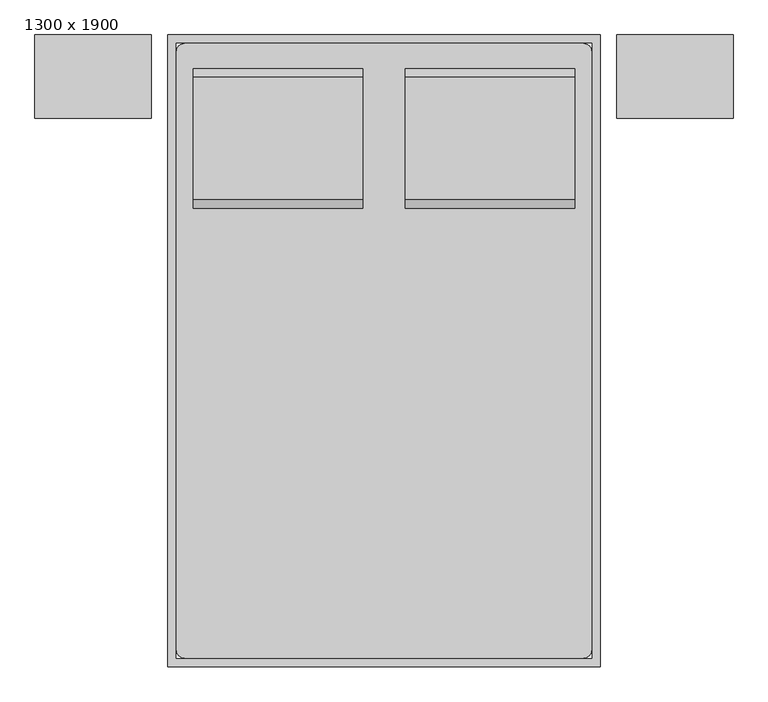
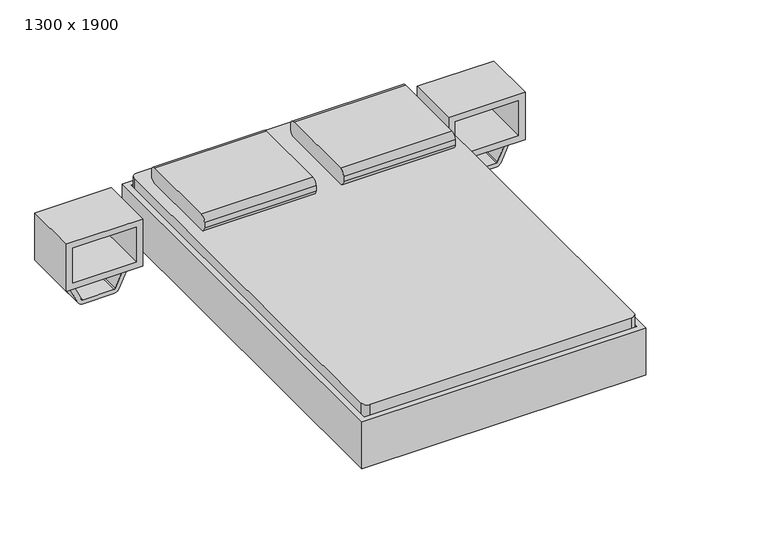
"""IFC4 building model written with IfcOpenShell, lengths in millimetres: furniture geometry, 双人床带床头柜 : 1300 x 1900."""

from ifc_helpers import new_model, si_unit, point, frame, frame_2d, origin, place, context, project, spatial, polyline, circle_curve, trimmed, segment, composite_curve, outline, extrude, source, transform, mapped, element, save
from ifc_brep_helpers import plane_surface, cylinder_surface, revolved_surface, advanced_brep


def furniture_1300_x_1900_48583a1e(model_context):
    return source(origin(), model_context, "Body", "SolidModel", [
        advanced_brep(
        [(-285.1231784, 461.5704918, 177.8), (-285.1231784, 385.3704918, 177.8), (-285.1231784, 385.3704918, 196.85), (-285.1231784, 461.5704918, 196.85), (-234.3231784, 461.5704918, 177.8), (-234.3231784, 385.3704918, 177.8), (-222.1869899, 385.3704918, 196.85), (-222.1869899, 461.5704918, 196.85), (-158.2523099, 461.5704918, 14.6654962), (-158.2523099, 385.3704918, 14.6654962), (-140.9871466, 385.3704918, 22.716374), (-140.9871466, 461.5704918, 22.716374), (-135.2320921, 385.3704918, 0.0), (-135.2320921, 461.5704918, 0.0), (-135.2320921, 385.3704918, 19.05), (-135.2320921, 461.5704918, 19.05), (-56.6195862, 461.5704918, 0.0), (-56.6195862, 385.3704918, 0.0), (-56.6195862, 385.3704918, 19.05), (-56.6195862, 461.5704918, 19.05), (-43.9195862, 385.3704918, 3.4029547), (-43.9195862, 461.5704918, 3.4029547), (-53.4445862, 385.3704918, 19.9007387), (-53.4445862, 461.5704918, 19.9007387), (16.177459, 461.5704918, 38.1), (16.177459, 385.3704918, 38.1), (11.0730269, 385.3704918, 57.15), (11.0730269, 461.5704918, 57.15), (662.4518216, 461.5704918, 38.1), (662.4518216, 385.3704918, 38.1), (667.5562537, 385.3704918, 57.15), (667.5562537, 461.5704918, 57.15), (722.5488669, 461.5704918, 3.4029547), (722.5488669, 385.3704918, 3.4029547), (732.0738669, 385.3704918, 19.9007387), (732.0738669, 461.5704918, 19.9007387), (735.2488669, 385.3704918, 0.0), (735.2488669, 461.5704918, 0.0), (735.2488669, 385.3704918, 19.05), (735.2488669, 461.5704918, 19.05), (813.8613728, 461.5704918, 0.0), (813.8613728, 385.3704918, 0.0), (813.8613728, 385.3704918, 19.05), (813.8613728, 461.5704918, 19.05), (836.8815906, 385.3704918, 14.6654962), (836.8815906, 461.5704918, 14.6654962), (819.6164272, 385.3704918, 22.716374), (819.6164272, 461.5704918, 22.716374), (912.952459, 461.5704918, 177.8), (912.952459, 385.3704918, 177.8), (900.8162705, 385.3704918, 196.85), (900.8162705, 461.5704918, 196.85), (963.752459, 461.5704918, 177.8), (963.752459, 461.5704918, 196.85), (963.752459, 385.3704918, 196.85), (963.752459, 385.3704918, 177.8)],
        [
            (0, 1),
            (1, 2),
            (2, 3),
            (3, 0),
            (0, 4),
            (4, 5),
            (5, 1),
            (5, 6),
            (6, 2),
            (6, 7),
            (7, 3),
            (7, 4),
            (4, 8),
            (8, 9),
            (9, 5),
            (9, 10),
            (10, 6),
            (10, 11),
            (11, 7),
            (11, 8),
            (12, 9, circle_curve(frame((-135.2320921, 385.3704918, 25.4), z_axis=(0.0, 1.0, 0.0), x_axis=(-0.9063077870366494, 0.0, -0.4226182617407007)), 25.4)),
            (8, 13, circle_curve(frame((-135.2320921, 461.5704918, 25.4), z_axis=(0.0, -1.0, 0.0), x_axis=(-0.9063077870366494, 0.0, -0.4226182617407007)), 25.4)),
            (13, 12),
            (14, 10, circle_curve(frame((-135.2320921, 385.3704918, 25.4), z_axis=(0.0, 1.0, 0.0), x_axis=(-0.9063077870366494, 0.0, -0.4226182617407007)), 6.35)),
            (12, 14),
            (15, 11, circle_curve(frame((-135.2320921, 461.5704918, 25.4), z_axis=(0.0, 1.0, 0.0), x_axis=(-0.9063077870366494, 0.0, -0.4226182617407007)), 6.35)),
            (14, 15),
            (15, 13),
            (13, 16),
            (16, 17),
            (17, 12),
            (17, 18),
            (18, 14),
            (18, 19),
            (19, 15),
            (19, 16),
            (20, 17, circle_curve(frame((-56.6195862, 385.3704918, 25.4), z_axis=(0.0, 1.0, 0.0), x_axis=(0.0, 0.0, -1.0)), 25.4)),
            (16, 21, circle_curve(frame((-56.6195862, 461.5704918, 25.4), z_axis=(0.0, -1.0, 0.0), x_axis=(0.0, 0.0, -1.0)), 25.4)),
            (21, 20),
            (22, 18, circle_curve(frame((-56.6195862, 385.3704918, 25.4), z_axis=(0.0, 1.0, 0.0), x_axis=(0.0, 0.0, -1.0)), 6.35)),
            (20, 22),
            (23, 19, circle_curve(frame((-56.6195862, 461.5704918, 25.4), z_axis=(0.0, 1.0, 0.0), x_axis=(0.0, 0.0, -1.0)), 6.35)),
            (22, 23),
            (23, 21),
            (21, 24),
            (24, 25),
            (25, 20),
            (25, 26),
            (26, 22),
            (26, 27),
            (27, 23),
            (27, 24),
            (24, 28),
            (28, 29),
            (29, 25),
            (29, 30),
            (30, 26),
            (30, 31),
            (31, 27),
            (31, 28),
            (28, 32),
            (32, 33),
            (33, 29),
            (33, 34),
            (34, 30),
            (34, 35),
            (35, 31),
            (35, 32),
            (36, 33, circle_curve(frame((735.2488669, 385.3704918, 25.4), z_axis=(0.0, 1.0, 0.0), x_axis=(-0.5000000000000505, 0.0, -0.8660254037844094)), 25.4)),
            (32, 37, circle_curve(frame((735.2488669, 461.5704918, 25.4), z_axis=(0.0, -1.0, 0.0), x_axis=(-0.5000000000000505, 0.0, -0.8660254037844094)), 25.4)),
            (37, 36),
            (38, 34, circle_curve(frame((735.2488669, 385.3704918, 25.4), z_axis=(0.0, 1.0, 0.0), x_axis=(-0.5000000000000505, 0.0, -0.8660254037844094)), 6.35)),
            (36, 38),
            (39, 35, circle_curve(frame((735.2488669, 461.5704918, 25.4), z_axis=(0.0, 1.0, 0.0), x_axis=(-0.5000000000000505, 0.0, -0.8660254037844094)), 6.35)),
            (38, 39),
            (39, 37),
            (37, 40),
            (40, 41),
            (41, 36),
            (41, 42),
            (42, 38),
            (42, 43),
            (43, 39),
            (43, 40),
            (44, 41, circle_curve(frame((813.8613728, 385.3704918, 25.4), z_axis=(0.0, 1.0, 0.0), x_axis=(0.0, 0.0, -1.0)), 25.4)),
            (40, 45, circle_curve(frame((813.8613728, 461.5704918, 25.4), z_axis=(0.0, -1.0, 0.0), x_axis=(0.0, 0.0, -1.0)), 25.4)),
            (45, 44),
            (46, 42, circle_curve(frame((813.8613728, 385.3704918, 25.4), z_axis=(0.0, 1.0, 0.0), x_axis=(0.0, 0.0, -1.0)), 6.35)),
            (44, 46),
            (47, 43, circle_curve(frame((813.8613728, 461.5704918, 25.4), z_axis=(0.0, 1.0, 0.0), x_axis=(0.0, 0.0, -1.0)), 6.35)),
            (46, 47),
            (47, 45),
            (45, 48),
            (48, 49),
            (49, 44),
            (49, 50),
            (50, 46),
            (50, 51),
            (51, 47),
            (51, 48),
            (52, 53),
            (53, 54),
            (54, 55),
            (55, 52),
            (48, 52),
            (55, 49),
            (54, 50),
            (53, 51),
        ],
        [
            plane_surface(frame((-285.1231784, 715.5704918, -152.9490627), z_axis=(-1.0, 0.0, 0.0), x_axis=(0.0, 1.0, 0.0))),
            plane_surface(frame((-285.1231784, 461.5704918, 177.8), z_axis=(0.0, 0.0, -1.0), x_axis=(1.0, 0.0, 0.0))),
            plane_surface(frame((-285.1231784, 385.3704918, 177.8), z_axis=(0.0, -1.0, 0.0), x_axis=(1.0, 0.0, 0.0))),
            plane_surface(frame((-285.1231784, 385.3704918, 196.85), z_axis=(0.0, 0.0, 1.0), x_axis=(1.0, 0.0, 0.0))),
            plane_surface(frame((-285.1231784, 461.5704918, 196.85), z_axis=(0.0, 1.0, 0.0), x_axis=(1.0, 0.0, 0.0))),
            plane_surface(frame((-234.3231784, 461.5704918, 177.8), z_axis=(-0.9063077870366483, 0.0, -0.42261826174070305), x_axis=(0.42261826174070305, 0.0, -0.9063077870366483))),
            plane_surface(frame((-234.3231784, 385.3704918, 177.8), z_axis=(0.0, -1.0, 0.0), x_axis=(0.4226182617407031, 0.0, -0.9063077870366483))),
            plane_surface(frame((-222.1869899, 385.3704918, 196.85), z_axis=(0.9063077870366483, 0.0, 0.42261826174070316), x_axis=(0.42261826174070316, 0.0, -0.9063077870366483))),
            plane_surface(frame((-222.1869899, 461.5704918, 196.85), z_axis=(0.0, 1.0, 0.0), x_axis=(0.42261826174070316, 0.0, -0.9063077870366483))),
            cylinder_surface(frame((-135.2320921, 715.5704918, 25.4), z_axis=(0.0, -1.0, 0.0), x_axis=(-0.9063077870366494, 0.0, -0.4226182617407007)), 25.4),
            plane_surface(frame((-135.2320921, 385.3704918, 25.4), z_axis=(0.0, -1.0, 0.0), x_axis=(-0.9063077870366494, 0.0, -0.4226182617407007))),
            revolved_surface(polyline([(-140.9871465476827, 385.3704918, 22.71637403794655), (-140.9871465476827, 461.5704918, 22.71637403794655)]), (-135.2320921, 715.5704918, 25.4), (0.0, -1.0, 0.0)),
            plane_surface(frame((-135.2320921, 461.5704918, 25.4), z_axis=(0.0, 1.0, 0.0), x_axis=(-0.9063077870366494, 0.0, -0.4226182617407007))),
            plane_surface(frame((-135.2320921, 461.5704918, 0.0), z_axis=(0.0, 0.0, -1.0), x_axis=(1.0, 0.0, 0.0))),
            plane_surface(frame((-135.2320921, 385.3704918, 0.0), z_axis=(0.0, -1.0, 0.0), x_axis=(1.0, 0.0, 0.0))),
            plane_surface(frame((-135.2320921, 385.3704918, 19.05), z_axis=(0.0, 0.0, 1.0), x_axis=(1.0, 0.0, 0.0))),
            plane_surface(frame((-135.2320921, 461.5704918, 19.05), z_axis=(0.0, 1.0, 0.0), x_axis=(1.0, 0.0, 0.0))),
            cylinder_surface(frame((-56.6195862, 715.5704918, 25.4), z_axis=(0.0, -1.0, 0.0), x_axis=(0.0, 0.0, -1.0)), 25.4),
            plane_surface(frame((-56.6195862, 385.3704918, 25.4), z_axis=(0.0, -1.0, 0.0), x_axis=(0.0, 0.0, -1.0))),
            revolved_surface(polyline([(-56.6195862, 385.3704918, 19.049999999999997), (-56.6195862, 461.5704918, 19.049999999999997)]), (-56.6195862, 715.5704918, 25.4), (0.0, -1.0, 0.0)),
            plane_surface(frame((-56.6195862, 461.5704918, 25.4), z_axis=(0.0, 1.0, 0.0), x_axis=(0.0, 0.0, -1.0))),
            plane_surface(frame((-43.9195862, 461.5704918, 3.4029547), z_axis=(0.49999999999987826, 0.0, -0.8660254037845089), x_axis=(0.8660254037845089, 0.0, 0.49999999999987826))),
            plane_surface(frame((-43.9195862, 385.3704918, 3.4029547), z_axis=(0.0, -1.0, 0.0), x_axis=(0.866025403784509, 0.0, 0.49999999999987815))),
            plane_surface(frame((-53.4445862, 385.3704918, 19.9007387), z_axis=(-0.49999999999987926, 0.0, 0.8660254037845083), x_axis=(0.8660254037845083, 0.0, 0.49999999999987926))),
            plane_surface(frame((-53.4445862, 461.5704918, 19.9007387), z_axis=(0.0, 1.0, 0.0), x_axis=(0.8660254037845087, 0.0, 0.4999999999998789))),
            plane_surface(frame((16.177459, 461.5704918, 38.1), z_axis=(0.0, 0.0, -1.0), x_axis=(1.0, 0.0, 0.0))),
            plane_surface(frame((16.177459, 385.3704918, 38.1), z_axis=(0.0, -1.0, 0.0), x_axis=(1.0, 0.0, 0.0))),
            plane_surface(frame((11.0730269, 385.3704918, 57.15), z_axis=(0.0, 0.0, 1.0), x_axis=(1.0, 0.0, 0.0))),
            plane_surface(frame((11.0730269, 461.5704918, 57.15), z_axis=(0.0, 1.0, 0.0), x_axis=(1.0, 0.0, 0.0))),
            plane_surface(frame((662.4518216, 461.5704918, 38.1), z_axis=(-0.5000000000000518, 0.0, -0.8660254037844087), x_axis=(0.8660254037844087, 0.0, -0.5000000000000518))),
            plane_surface(frame((662.4518216, 385.3704918, 38.1), z_axis=(0.0, -1.0, 0.0), x_axis=(0.8660254037844093, 0.0, -0.500000000000051))),
            plane_surface(frame((667.5562537, 385.3704918, 57.15), z_axis=(0.5000000000000507, 0.0, 0.8660254037844094), x_axis=(0.8660254037844094, 0.0, -0.5000000000000507))),
            plane_surface(frame((667.5562537, 461.5704918, 57.15), z_axis=(0.0, 1.0000000000000002, 0.0), x_axis=(0.8660254037844094, 0.0, -0.5000000000000508))),
            cylinder_surface(frame((735.2488669, 715.5704918, 25.4), z_axis=(0.0, -1.0, 0.0), x_axis=(-0.5000000000000505, 0.0, -0.8660254037844094)), 25.4),
            plane_surface(frame((735.2488669, 385.3704918, 25.4), z_axis=(0.0, -1.0, 0.0), x_axis=(-0.5000000000000506, 0.0, -0.8660254037844095))),
            revolved_surface(polyline([(732.0738668999998, 385.3704918, 19.900738685969), (732.0738668999998, 461.5704918, 19.900738685969)]), (735.2488669, 715.5704918, 25.4), (0.0, -1.0, 0.0)),
            plane_surface(frame((735.2488669, 461.5704918, 25.4), z_axis=(0.0, 1.0, 0.0), x_axis=(-0.5000000000000506, 0.0, -0.8660254037844095))),
            plane_surface(frame((735.2488669, 461.5704918, 0.0), z_axis=(0.0, 0.0, -1.0), x_axis=(1.0, 0.0, 0.0))),
            plane_surface(frame((735.2488669, 385.3704918, 0.0), z_axis=(0.0, -1.0, 0.0), x_axis=(1.0, 0.0, 0.0))),
            plane_surface(frame((735.2488669, 385.3704918, 19.05), z_axis=(0.0, 0.0, 1.0), x_axis=(1.0, 0.0, 0.0))),
            plane_surface(frame((735.2488669, 461.5704918, 19.05), z_axis=(0.0, 1.0, 0.0), x_axis=(1.0, 0.0, 0.0))),
            cylinder_surface(frame((813.8613728, 715.5704918, 25.4), z_axis=(0.0, -1.0, 0.0), x_axis=(0.0, 0.0, -1.0)), 25.4),
            plane_surface(frame((813.8613728, 385.3704918, 25.4), z_axis=(0.0, -1.0, 0.0), x_axis=(0.0, 0.0, -1.0))),
            revolved_surface(polyline([(813.8613728, 385.3704918, 19.049999999999997), (813.8613728, 461.5704918, 19.049999999999997)]), (813.8613728, 715.5704918, 25.4), (0.0, -1.0, 0.0)),
            plane_surface(frame((813.8613728, 461.5704918, 25.4), z_axis=(0.0, 1.0, 0.0), x_axis=(0.0, 0.0, -1.0))),
            plane_surface(frame((836.8815906, 461.5704918, 14.6654962), z_axis=(0.9063077870366775, 0.0, -0.42261826174064077), x_axis=(0.42261826174064077, 0.0, 0.9063077870366775))),
            plane_surface(frame((836.8815906, 385.3704918, 14.6654962), z_axis=(0.0, -1.0, 0.0), x_axis=(0.42261826174063993, 0.0, 0.9063077870366777))),
            plane_surface(frame((819.6164272, 385.3704918, 22.716374), z_axis=(-0.9063077870366776, 0.0, 0.4226182617406402), x_axis=(0.4226182617406402, 0.0, 0.9063077870366776))),
            plane_surface(frame((819.6164272, 461.5704918, 22.716374), z_axis=(0.0, 1.0, 0.0), x_axis=(0.4226182617406405, 0.0, 0.9063077870366775))),
            plane_surface(frame((963.752459, 715.5704918, -152.9490627), z_axis=(1.0, 0.0, 0.0), x_axis=(0.0, 1.0, 0.0))),
            plane_surface(frame((912.952459, 461.5704918, 177.8), z_axis=(0.0, 0.0, -1.0), x_axis=(1.0, 0.0, 0.0))),
            plane_surface(frame((912.952459, 385.3704918, 177.8), z_axis=(0.0, -1.0, 0.0), x_axis=(1.0, 0.0, 0.0))),
            plane_surface(frame((900.8162705, 385.3704918, 196.85), z_axis=(0.0, 0.0, 1.0), x_axis=(1.0, 0.0, 0.0))),
            plane_surface(frame((900.8162705, 461.5704918, 196.85), z_axis=(0.0, 1.0, 0.0), x_axis=(1.0, 0.0, 0.0))),
        ],
        [
            (0, [[1, 2, 3, 4]]),
            (1, [[-1, 5, 6, 7]]),
            (2, [[-2, -7, 8, 9]]),
            (3, [[-3, -9, 10, 11]]),
            (4, [[-4, -11, 12, -5]]),
            (5, [[-6, 13, 14, 15]]),
            (6, [[-8, -15, 16, 17]]),
            (7, [[-10, -17, 18, 19]]),
            (8, [[-12, -19, 20, -13]]),
            (9, [[21, -14, 22, 23]]),
            (10, [[24, -16, -21, 25]]),
            (11, [[26, -18, -24, 27]]),
            (12, [[-22, -20, -26, 28]]),
            (13, [[-23, 29, 30, 31]]),
            (14, [[-25, -31, 32, 33]]),
            (15, [[-27, -33, 34, 35]]),
            (16, [[-28, -35, 36, -29]]),
            (17, [[37, -30, 38, 39]]),
            (18, [[40, -32, -37, 41]]),
            (19, [[42, -34, -40, 43]]),
            (20, [[-38, -36, -42, 44]]),
            (21, [[-39, 45, 46, 47]]),
            (22, [[-41, -47, 48, 49]]),
            (23, [[-43, -49, 50, 51]]),
            (24, [[-44, -51, 52, -45]]),
            (25, [[-46, 53, 54, 55]]),
            (26, [[-48, -55, 56, 57]]),
            (27, [[-50, -57, 58, 59]]),
            (28, [[-52, -59, 60, -53]]),
            (29, [[-54, 61, 62, 63]]),
            (30, [[-56, -63, 64, 65]]),
            (31, [[-58, -65, 66, 67]]),
            (32, [[-60, -67, 68, -61]]),
            (33, [[69, -62, 70, 71]]),
            (34, [[72, -64, -69, 73]]),
            (35, [[74, -66, -72, 75]]),
            (36, [[-70, -68, -74, 76]]),
            (37, [[-71, 77, 78, 79]]),
            (38, [[-73, -79, 80, 81]]),
            (39, [[-75, -81, 82, 83]]),
            (40, [[-76, -83, 84, -77]]),
            (41, [[85, -78, 86, 87]]),
            (42, [[88, -80, -85, 89]]),
            (43, [[90, -82, -88, 91]]),
            (44, [[-86, -84, -90, 92]]),
            (45, [[-87, 93, 94, 95]]),
            (46, [[-89, -95, 96, 97]]),
            (47, [[-91, -97, 98, 99]]),
            (48, [[-92, -99, 100, -93]]),
            (49, [[101, 102, 103, 104]]),
            (50, [[-94, 105, -104, 106]]),
            (51, [[-96, -106, -103, 107]]),
            (52, [[-98, -107, -102, 108]]),
            (53, [[-100, -108, -101, -105]]),
        ],
    ),
        advanced_brep(
        [(-285.447541, -879.6295082, 196.85), (-285.447541, -879.6295082, 177.8), (-285.447541, -955.8295082, 177.8), (-285.447541, -955.8295082, 196.85), (-222.5113525, -879.6295082, 196.85), (-234.647541, -879.6295082, 177.8), (-234.647541, -955.8295082, 177.8), (-222.5113525, -955.8295082, 196.85), (-141.3115092, -879.6295082, 22.716374), (-158.5766725, -879.6295082, 14.6654962), (-158.5766725, -955.8295082, 14.6654962), (-141.3115092, -955.8295082, 22.716374), (-135.5564547, -879.6295082, 0.0), (-135.5564547, -879.6295082, 19.05), (-135.5564547, -955.8295082, 0.0), (-135.5564547, -955.8295082, 19.05), (-56.9439489, -879.6295082, 19.05), (-56.9439489, -879.6295082, 0.0), (-56.9439489, -955.8295082, 0.0), (-56.9439489, -955.8295082, 19.05), (-44.2439489, -879.6295082, 3.4029547), (-53.7689489, -879.6295082, 19.9007387), (-44.2439489, -955.8295082, 3.4029547), (-53.7689489, -955.8295082, 19.9007387), (10.7486643, -879.6295082, 57.15), (15.8530964, -879.6295082, 38.1), (15.8530964, -955.8295082, 38.1), (10.7486643, -955.8295082, 57.15), (667.5562537, -879.6295082, 57.15), (662.4518216, -879.6295082, 38.1), (662.4518216, -955.8295082, 38.1), (667.5562537, -955.8295082, 57.15), (732.0738669, -879.6295082, 19.9007387), (722.5488669, -879.6295082, 3.4029547), (722.5488669, -955.8295082, 3.4029547), (732.0738669, -955.8295082, 19.9007387), (735.2488669, -879.6295082, 0.0), (735.2488669, -879.6295082, 19.05), (735.2488669, -955.8295082, 0.0), (735.2488669, -955.8295082, 19.05), (813.8613728, -879.6295082, 19.05), (813.8613728, -879.6295082, 0.0), (813.8613728, -955.8295082, 0.0), (813.8613728, -955.8295082, 19.05), (836.8815906, -879.6295082, 14.6654962), (819.6164272, -879.6295082, 22.716374), (836.8815906, -955.8295082, 14.6654962), (819.6164272, -955.8295082, 22.716374), (900.8162705, -879.6295082, 196.85), (912.952459, -879.6295082, 177.8), (912.952459, -955.8295082, 177.8), (900.8162705, -955.8295082, 196.85), (963.752459, -879.6295082, 196.85), (963.752459, -955.8295082, 196.85), (963.752459, -955.8295082, 177.8), (963.752459, -879.6295082, 177.8)],
        [
            (0, 1),
            (1, 2),
            (2, 3),
            (3, 0),
            (0, 4),
            (4, 5),
            (5, 1),
            (5, 6),
            (6, 2),
            (6, 7),
            (7, 3),
            (7, 4),
            (4, 8),
            (8, 9),
            (9, 5),
            (9, 10),
            (10, 6),
            (10, 11),
            (11, 7),
            (11, 8),
            (12, 9, circle_curve(frame((-135.5564547, -879.6295082, 25.4), z_axis=(0.0, 1.0, 0.0), x_axis=(-0.9063077870366627, 0.0, -0.42261826174067213)), 25.4)),
            (8, 13, circle_curve(frame((-135.5564547, -879.6295082, 25.4), z_axis=(0.0, -1.0, 0.0), x_axis=(-0.9063077870366627, 0.0, -0.42261826174067213)), 6.35)),
            (13, 12),
            (14, 10, circle_curve(frame((-135.5564547, -955.8295082, 25.4), z_axis=(0.0, 1.0, 0.0), x_axis=(-0.9063077870366627, 0.0, -0.42261826174067213)), 25.4)),
            (12, 14),
            (15, 11, circle_curve(frame((-135.5564547, -955.8295082, 25.4), z_axis=(0.0, 1.0, 0.0), x_axis=(-0.9063077870366627, 0.0, -0.42261826174067213)), 6.35)),
            (14, 15),
            (15, 13),
            (13, 16),
            (16, 17),
            (17, 12),
            (17, 18),
            (18, 14),
            (18, 19),
            (19, 15),
            (19, 16),
            (20, 17, circle_curve(frame((-56.9439489, -879.6295082, 25.4), z_axis=(0.0, 1.0, 0.0), x_axis=(0.0, 0.0, -1.0)), 25.4)),
            (16, 21, circle_curve(frame((-56.9439489, -879.6295082, 25.4), z_axis=(0.0, -1.0, 0.0), x_axis=(0.0, 0.0, -1.0)), 6.35)),
            (21, 20),
            (22, 18, circle_curve(frame((-56.9439489, -955.8295082, 25.4), z_axis=(0.0, 1.0, 0.0), x_axis=(0.0, 0.0, -1.0)), 25.4)),
            (20, 22),
            (23, 19, circle_curve(frame((-56.9439489, -955.8295082, 25.4), z_axis=(0.0, 1.0, 0.0), x_axis=(0.0, 0.0, -1.0)), 6.35)),
            (22, 23),
            (23, 21),
            (21, 24),
            (24, 25),
            (25, 20),
            (25, 26),
            (26, 22),
            (26, 27),
            (27, 23),
            (27, 24),
            (24, 28),
            (28, 29),
            (29, 25),
            (29, 30),
            (30, 26),
            (30, 31),
            (31, 27),
            (31, 28),
            (28, 32),
            (32, 33),
            (33, 29),
            (33, 34),
            (34, 30),
            (34, 35),
            (35, 31),
            (35, 32),
            (36, 33, circle_curve(frame((735.2488669, -879.6295082, 25.4), z_axis=(0.0, 1.0, 0.0), x_axis=(-0.5000000000000517, 0.0, -0.8660254037844087)), 25.4)),
            (32, 37, circle_curve(frame((735.2488669, -879.6295082, 25.4), z_axis=(0.0, -1.0, 0.0), x_axis=(-0.5000000000000517, 0.0, -0.8660254037844087)), 6.35)),
            (37, 36),
            (38, 34, circle_curve(frame((735.2488669, -955.8295082, 25.4), z_axis=(0.0, 1.0, 0.0), x_axis=(-0.5000000000000517, 0.0, -0.8660254037844087)), 25.4)),
            (36, 38),
            (39, 35, circle_curve(frame((735.2488669, -955.8295082, 25.4), z_axis=(0.0, 1.0, 0.0), x_axis=(-0.5000000000000517, 0.0, -0.8660254037844087)), 6.35)),
            (38, 39),
            (39, 37),
            (37, 40),
            (40, 41),
            (41, 36),
            (41, 42),
            (42, 38),
            (42, 43),
            (43, 39),
            (43, 40),
            (44, 41, circle_curve(frame((813.8613728, -879.6295082, 25.4), z_axis=(0.0, 1.0, 0.0), x_axis=(0.0, 0.0, -1.0)), 25.4)),
            (40, 45, circle_curve(frame((813.8613728, -879.6295082, 25.4), z_axis=(0.0, -1.0, 0.0), x_axis=(0.0, 0.0, -1.0)), 6.35)),
            (45, 44),
            (46, 42, circle_curve(frame((813.8613728, -955.8295082, 25.4), z_axis=(0.0, 1.0, 0.0), x_axis=(0.0, 0.0, -1.0)), 25.4)),
            (44, 46),
            (47, 43, circle_curve(frame((813.8613728, -955.8295082, 25.4), z_axis=(0.0, 1.0, 0.0), x_axis=(0.0, 0.0, -1.0)), 6.35)),
            (46, 47),
            (47, 45),
            (45, 48),
            (48, 49),
            (49, 44),
            (49, 50),
            (50, 46),
            (50, 51),
            (51, 47),
            (51, 48),
            (52, 53),
            (53, 54),
            (54, 55),
            (55, 52),
            (48, 52),
            (55, 49),
            (54, 50),
            (53, 51),
        ],
        [
            plane_surface(frame((-285.447541, -1184.4295082, -127.5947323), z_axis=(-1.0, 0.0, 0.0), x_axis=(0.0, 1.0, 0.0))),
            plane_surface(frame((-285.447541, -879.6295082, 196.85), z_axis=(0.0, 1.0, 0.0), x_axis=(1.0, 0.0, 0.0))),
            plane_surface(frame((-285.447541, -879.6295082, 177.8), z_axis=(0.0, 0.0, -1.0), x_axis=(1.0, 0.0, 0.0))),
            plane_surface(frame((-285.447541, -955.8295082, 177.8), z_axis=(0.0, -1.0, 0.0), x_axis=(1.0, 0.0, 0.0))),
            plane_surface(frame((-285.447541, -955.8295082, 196.85), z_axis=(0.0, 0.0, 1.0), x_axis=(1.0, 0.0, 0.0))),
            plane_surface(frame((-222.5113525, -879.6295082, 196.85), z_axis=(0.0, 1.0, 0.0), x_axis=(0.42261826174067113, 0.0, -0.9063077870366631))),
            plane_surface(frame((-234.647541, -879.6295082, 177.8), z_axis=(-0.9063077870366633, 0.0, -0.422618261740671), x_axis=(0.422618261740671, 0.0, -0.9063077870366633))),
            plane_surface(frame((-234.647541, -955.8295082, 177.8), z_axis=(0.0, -1.0, 0.0), x_axis=(0.422618261740671, 0.0, -0.9063077870366633))),
            plane_surface(frame((-222.5113525, -955.8295082, 196.85), z_axis=(0.9063077870366631, 0.0, 0.42261826174067113), x_axis=(0.42261826174067113, 0.0, -0.9063077870366631))),
            plane_surface(frame((-135.5564547, -879.6295082, 25.4), z_axis=(0.0, 1.0, 0.0), x_axis=(-0.9063077870366627, 0.0, -0.42261826174067213))),
            cylinder_surface(frame((-135.5564547, -1184.4295082, 25.4), z_axis=(0.0, -1.0, 0.0), x_axis=(-0.9063077870366627, 0.0, -0.42261826174067213)), 25.4),
            plane_surface(frame((-135.5564547, -955.8295082, 25.4), z_axis=(0.0, -1.0, 0.0), x_axis=(-0.9063077870366627, 0.0, -0.42261826174067213))),
            revolved_surface(polyline([(-141.31150914768278, -955.8295082, 22.716374037946732), (-141.31150914768278, -879.6295082, 22.716374037946732)]), (-135.5564547, -1184.4295082, 25.4), (0.0, -1.0, 0.0)),
            plane_surface(frame((-135.5564547, -879.6295082, 19.05), z_axis=(0.0, 1.0, 0.0), x_axis=(1.0, 0.0, 0.0))),
            plane_surface(frame((-135.5564547, -879.6295082, 0.0), z_axis=(0.0, 0.0, -1.0), x_axis=(1.0, 0.0, 0.0))),
            plane_surface(frame((-135.5564547, -955.8295082, 0.0), z_axis=(0.0, -1.0, 0.0), x_axis=(1.0, 0.0, 0.0))),
            plane_surface(frame((-135.5564547, -955.8295082, 19.05), z_axis=(0.0, 0.0, 1.0), x_axis=(1.0, 0.0, 0.0))),
            plane_surface(frame((-56.9439489, -879.6295082, 25.4), z_axis=(0.0, 1.0, 0.0), x_axis=(0.0, 0.0, -1.0))),
            cylinder_surface(frame((-56.9439489, -1184.4295082, 25.4), z_axis=(0.0, -1.0, 0.0), x_axis=(0.0, 0.0, -1.0)), 25.4),
            plane_surface(frame((-56.9439489, -955.8295082, 25.4), z_axis=(0.0, -1.0, 0.0), x_axis=(0.0, 0.0, -1.0))),
            revolved_surface(polyline([(-56.9439489, -955.8295082, 19.049999999999997), (-56.9439489, -879.6295082, 19.049999999999997)]), (-56.9439489, -1184.4295082, 25.4), (0.0, -1.0, 0.0)),
            plane_surface(frame((-53.7689489, -879.6295082, 19.9007387), z_axis=(0.0, 1.0, 0.0), x_axis=(0.8660254037844793, 0.0, 0.4999999999999296))),
            plane_surface(frame((-44.2439489, -879.6295082, 3.4029547), z_axis=(0.4999999999999292, 0.0, -0.8660254037844796), x_axis=(0.8660254037844796, 0.0, 0.4999999999999292))),
            plane_surface(frame((-44.2439489, -955.8295082, 3.4029547), z_axis=(0.0, -1.0000000000000002, 0.0), x_axis=(0.8660254037844802, 0.0, 0.4999999999999281))),
            plane_surface(frame((-53.7689489, -955.8295082, 19.9007387), z_axis=(-0.49999999999992867, 0.0, 0.8660254037844798), x_axis=(0.8660254037844798, 0.0, 0.49999999999992867))),
            plane_surface(frame((10.7486643, -879.6295082, 57.15), z_axis=(0.0, 1.0, 0.0), x_axis=(1.0, 0.0, 0.0))),
            plane_surface(frame((15.8530964, -879.6295082, 38.1), z_axis=(0.0, 0.0, -1.0), x_axis=(1.0, 0.0, 0.0))),
            plane_surface(frame((15.8530964, -955.8295082, 38.1), z_axis=(0.0, -1.0, 0.0), x_axis=(1.0, 0.0, 0.0))),
            plane_surface(frame((10.7486643, -955.8295082, 57.15), z_axis=(0.0, 0.0, 1.0), x_axis=(1.0, 0.0, 0.0))),
            plane_surface(frame((667.5562537, -879.6295082, 57.15), z_axis=(0.0, 1.0, 0.0), x_axis=(0.8660254037844098, 0.0, -0.50000000000005))),
            plane_surface(frame((662.4518216, -879.6295082, 38.1), z_axis=(-0.5000000000000507, 0.0, -0.8660254037844094), x_axis=(0.8660254037844094, 0.0, -0.5000000000000507))),
            plane_surface(frame((662.4518216, -955.8295082, 38.1), z_axis=(0.0, -1.0000000000000002, 0.0), x_axis=(0.8660254037844093, 0.0, -0.5000000000000511))),
            plane_surface(frame((667.5562537, -955.8295082, 57.15), z_axis=(0.5000000000000511, 0.0, 0.8660254037844092), x_axis=(0.8660254037844092, 0.0, -0.5000000000000511))),
            plane_surface(frame((735.2488669, -879.6295082, 25.4), z_axis=(0.0, 1.0000000000000002, 0.0), x_axis=(-0.5000000000000518, 0.0, -0.8660254037844088))),
            cylinder_surface(frame((735.2488669, -1184.4295082, 25.4), z_axis=(0.0, -1.0, 0.0), x_axis=(-0.5000000000000517, 0.0, -0.8660254037844087)), 25.4),
            plane_surface(frame((735.2488669, -955.8295082, 25.4), z_axis=(0.0, -1.0000000000000002, 0.0), x_axis=(-0.5000000000000518, 0.0, -0.8660254037844088))),
            revolved_surface(polyline([(732.0738668999998, -955.8295082, 19.900738685969003), (732.0738668999998, -879.6295082, 19.900738685969003)]), (735.2488669, -1184.4295082, 25.4), (0.0, -1.0, 0.0)),
            plane_surface(frame((735.2488669, -879.6295082, 19.05), z_axis=(0.0, 1.0, 0.0), x_axis=(1.0, 0.0, 0.0))),
            plane_surface(frame((735.2488669, -879.6295082, 0.0), z_axis=(0.0, 0.0, -1.0), x_axis=(1.0, 0.0, 0.0))),
            plane_surface(frame((735.2488669, -955.8295082, 0.0), z_axis=(0.0, -1.0, 0.0), x_axis=(1.0, 0.0, 0.0))),
            plane_surface(frame((735.2488669, -955.8295082, 19.05), z_axis=(0.0, 0.0, 1.0), x_axis=(1.0, 0.0, 0.0))),
            plane_surface(frame((813.8613728, -879.6295082, 25.4), z_axis=(0.0, 1.0, 0.0), x_axis=(0.0, 0.0, -1.0))),
            cylinder_surface(frame((813.8613728, -1184.4295082, 25.4), z_axis=(0.0, -1.0, 0.0), x_axis=(0.0, 0.0, -1.0)), 25.4),
            plane_surface(frame((813.8613728, -955.8295082, 25.4), z_axis=(0.0, -1.0, 0.0), x_axis=(0.0, 0.0, -1.0))),
            revolved_surface(polyline([(813.8613728, -955.8295082, 19.049999999999997), (813.8613728, -879.6295082, 19.049999999999997)]), (813.8613728, -1184.4295082, 25.4), (0.0, -1.0, 0.0)),
            plane_surface(frame((819.6164272, -879.6295082, 22.716374), z_axis=(0.0, 1.0, 0.0), x_axis=(0.4226182617405424, 0.0, 0.9063077870367232))),
            plane_surface(frame((836.8815906, -879.6295082, 14.6654962), z_axis=(0.9063077870367232, 0.0, -0.42261826174054246), x_axis=(0.42261826174054246, 0.0, 0.9063077870367232))),
            plane_surface(frame((836.8815906, -955.8295082, 14.6654962), z_axis=(0.0, -1.0, 0.0), x_axis=(0.4226182617405424, 0.0, 0.9063077870367232))),
            plane_surface(frame((819.6164272, -955.8295082, 22.716374), z_axis=(-0.906307787036723, 0.0, 0.42261826174054284), x_axis=(0.42261826174054284, 0.0, 0.906307787036723))),
            plane_surface(frame((963.752459, -1184.4295082, -127.5947323), z_axis=(1.0, 0.0, 0.0), x_axis=(0.0, 1.0, 0.0))),
            plane_surface(frame((900.8162705, -879.6295082, 196.85), z_axis=(0.0, 1.0, 0.0), x_axis=(1.0, 0.0, 0.0))),
            plane_surface(frame((912.952459, -879.6295082, 177.8), z_axis=(0.0, 0.0, -1.0), x_axis=(1.0, 0.0, 0.0))),
            plane_surface(frame((912.952459, -955.8295082, 177.8), z_axis=(0.0, -1.0, 0.0), x_axis=(1.0, 0.0, 0.0))),
            plane_surface(frame((900.8162705, -955.8295082, 196.85), z_axis=(0.0, 0.0, 1.0), x_axis=(1.0, 0.0, 0.0))),
        ],
        [
            (0, [[1, 2, 3, 4]]),
            (1, [[-1, 5, 6, 7]]),
            (2, [[-2, -7, 8, 9]]),
            (3, [[-3, -9, 10, 11]]),
            (4, [[-4, -11, 12, -5]]),
            (5, [[-6, 13, 14, 15]]),
            (6, [[-8, -15, 16, 17]]),
            (7, [[-10, -17, 18, 19]]),
            (8, [[-12, -19, 20, -13]]),
            (9, [[21, -14, 22, 23]]),
            (10, [[24, -16, -21, 25]]),
            (11, [[26, -18, -24, 27]]),
            (12, [[-22, -20, -26, 28]]),
            (13, [[-23, 29, 30, 31]]),
            (14, [[-25, -31, 32, 33]]),
            (15, [[-27, -33, 34, 35]]),
            (16, [[-28, -35, 36, -29]]),
            (17, [[37, -30, 38, 39]]),
            (18, [[40, -32, -37, 41]]),
            (19, [[42, -34, -40, 43]]),
            (20, [[-38, -36, -42, 44]]),
            (21, [[-39, 45, 46, 47]]),
            (22, [[-41, -47, 48, 49]]),
            (23, [[-43, -49, 50, 51]]),
            (24, [[-44, -51, 52, -45]]),
            (25, [[-46, 53, 54, 55]]),
            (26, [[-48, -55, 56, 57]]),
            (27, [[-50, -57, 58, 59]]),
            (28, [[-52, -59, 60, -53]]),
            (29, [[-54, 61, 62, 63]]),
            (30, [[-56, -63, 64, 65]]),
            (31, [[-58, -65, 66, 67]]),
            (32, [[-60, -67, 68, -61]]),
            (33, [[69, -62, 70, 71]]),
            (34, [[72, -64, -69, 73]]),
            (35, [[74, -66, -72, 75]]),
            (36, [[-70, -68, -74, 76]]),
            (37, [[-71, 77, 78, 79]]),
            (38, [[-73, -79, 80, 81]]),
            (39, [[-75, -81, 82, 83]]),
            (40, [[-76, -83, 84, -77]]),
            (41, [[85, -78, 86, 87]]),
            (42, [[88, -80, -85, 89]]),
            (43, [[90, -82, -88, 91]]),
            (44, [[-86, -84, -90, 92]]),
            (45, [[-87, 93, 94, 95]]),
            (46, [[-89, -95, 96, 97]]),
            (47, [[-91, -97, 98, 99]]),
            (48, [[-92, -99, 100, -93]]),
            (49, [[101, 102, 103, 104]]),
            (50, [[-94, 105, -104, 106]]),
            (51, [[-96, -106, -103, 107]]),
            (52, [[-98, -107, -102, 108]]),
            (53, [[-100, -108, -101, -105]]),
        ],
    ),
        extrude(outline(composite_curve([segment(polyline([(588.5704918, 406.4), (220.2704918, 406.4)]), True, "CONTINUOUS"), segment(trimmed(circle_curve(frame_2d((220.2704918, 431.8)), 25.4), [point((220.2704918, 406.4))], [point((194.8704918, 431.8))], False, "CARTESIAN"), True, "CONTINUOUS"), segment(polyline([(194.8704918, 431.8), (194.8704918, 457.2)]), True, "CONTINUOUS"), segment(trimmed(circle_curve(frame_2d((220.2704918, 457.2)), 25.4), [point((194.8704918, 457.2))], [point((220.2704918, 482.6))], False, "CARTESIAN"), True, "CONTINUOUS"), segment(polyline([(220.2704918, 482.6), (588.5704918, 482.6)]), True, "CONTINUOUS"), segment(trimmed(circle_curve(frame_2d((588.5704918, 457.2)), 25.4), [point((588.5704918, 482.6))], [point((613.9704918, 457.2))], False, "CARTESIAN"), True, "CONTINUOUS"), segment(polyline([(613.9704918, 457.2), (613.9704918, 431.8)]), True, "CONTINUOUS"), segment(trimmed(circle_curve(frame_2d((588.5704918, 431.8)), 25.4), [point((613.9704918, 431.8))], [point((588.5704918, 406.4))], False, "CARTESIAN"), True, "CONTINUOUS")], self_intersect=False)), frame((402.652459, 0.0, 0.0), z_axis=(1.0, 0.0, 0.0), x_axis=(0.0, 1.0, 0.0)), (0.0, 0.0, 1.0), 510.3),
        extrude(outline(composite_curve([segment(polyline([(588.5704918, 406.4), (220.2704918, 406.4)]), True, "CONTINUOUS"), segment(trimmed(circle_curve(frame_2d((220.2704918, 431.8)), 25.4), [point((220.2704918, 406.4))], [point((194.8704918, 431.8))], False, "CARTESIAN"), True, "CONTINUOUS"), segment(polyline([(194.8704918, 431.8), (194.8704918, 457.2)]), True, "CONTINUOUS"), segment(trimmed(circle_curve(frame_2d((220.2704918, 457.2)), 25.4), [point((194.8704918, 457.2))], [point((220.2704918, 482.6))], False, "CARTESIAN"), True, "CONTINUOUS"), segment(polyline([(220.2704918, 482.6), (588.5704918, 482.6)]), True, "CONTINUOUS"), segment(trimmed(circle_curve(frame_2d((588.5704918, 457.2)), 25.4), [point((588.5704918, 482.6))], [point((613.9704918, 457.2))], False, "CARTESIAN"), True, "CONTINUOUS"), segment(polyline([(613.9704918, 457.2), (613.9704918, 431.8)]), True, "CONTINUOUS"), segment(trimmed(circle_curve(frame_2d((588.5704918, 431.8)), 25.4), [point((613.9704918, 431.8))], [point((588.5704918, 406.4))], False, "CARTESIAN"), True, "CONTINUOUS")], self_intersect=False)), frame((-234.647541, 0.0, 0.0), z_axis=(1.0, 0.0, 0.0), x_axis=(0.0, 1.0, 0.0)), (0.0, 0.0, 1.0), 510.3),
        extrude(outline(composite_curve([segment(polyline([(-260.047541, 690.1704918), (938.352459, 690.1704918)]), True, "CONTINUOUS"), segment(trimmed(circle_curve(frame_2d((938.352459, 664.7704918)), 25.4), [point((938.352459, 690.1704918))], [point((963.752459, 664.7704918))], False, "CARTESIAN"), True, "CONTINUOUS"), segment(polyline([(963.752459, 664.7704918), (963.752459, -1133.6295082)]), True, "CONTINUOUS"), segment(trimmed(circle_curve(frame_2d((938.352459, -1133.6295082)), 25.4), [point((963.752459, -1133.6295082))], [point((938.352459, -1159.0295082))], False, "CARTESIAN"), True, "CONTINUOUS"), segment(polyline([(938.352459, -1159.0295082), (-260.047541, -1159.0295082)]), True, "CONTINUOUS"), segment(trimmed(circle_curve(frame_2d((-260.047541, -1133.6295082)), 25.4), [point((-260.047541, -1159.0295082))], [point((-285.447541, -1133.6295082))], False, "CARTESIAN"), True, "CONTINUOUS"), segment(polyline([(-285.447541, -1133.6295082), (-285.447541, 664.7704918)]), True, "CONTINUOUS"), segment(trimmed(circle_curve(frame_2d((-260.047541, 664.7704918)), 25.4), [point((-285.447541, 664.7704918))], [point((-260.047541, 690.1704918))], False, "CARTESIAN"), True, "CONTINUOUS")], self_intersect=False)), frame((0.0, 0.0, 203.2), z_axis=(0.0, 0.0, 1.0), x_axis=(1.0, 0.0, 0.0)), (0.0, 0.0, 1.0), 203.2),
        extrude(outline(composite_curve([segment(polyline([(14.6654962, -441.7035367), (116.2774654, -394.3210972), (127.0, -394.3210972), (127.0, -414.3210972), (118.4634671, -414.3210972), (22.716374, -458.9687)]), True, "CONTINUOUS"), segment(trimmed(circle_curve(frame_2d((25.4, -464.7237544)), 6.35), [point((22.716374, -458.9687))], [point((19.05, -464.7237544))], True, "CARTESIAN"), True, "CONTINUOUS"), segment(polyline([(19.05, -464.7237544), (19.05, -606.9713275)]), True, "CONTINUOUS"), segment(trimmed(circle_curve(frame_2d((25.4, -606.9713275)), 6.35), [point((19.05, -606.9713275))], [point((22.716374, -612.726382))], True, "CARTESIAN"), True, "CONTINUOUS"), segment(polyline([(22.716374, -612.726382), (118.4634671, -657.3739847), (127.0, -657.3739847), (127.0, -677.3739847), (116.2774654, -677.3739847), (14.6654962, -629.9915453)]), True, "CONTINUOUS"), segment(trimmed(circle_curve(frame_2d((25.4, -606.9713275)), 25.4), [point((14.6654962, -629.9915453))], [point((0.0, -606.9713275))], False, "CARTESIAN"), True, "CONTINUOUS"), segment(polyline([(0.0, -606.9713275), (0.0, -464.7237544)]), True, "CONTINUOUS"), segment(trimmed(circle_curve(frame_2d((25.4, -464.7237544)), 25.4), [point((0.0, -464.7237544))], [point((14.6654962, -441.7035367))], False, "CARTESIAN"), True, "CONTINUOUS")], self_intersect=False)), frame((0.0, 515.5704918, 0.0), z_axis=(0.0, 1.0, 0.0), x_axis=(0.0, 0.0, 1.0)), (0.0, 0.0, 1.0), 150.0),
        extrude(outline(polyline([(127.0, -360.847541), (355.6, -360.847541), (355.6, -710.847541), (127.0, -710.847541), (127.0, -360.847541)]), holes=[polyline([(325.6, -680.847541), (325.6, -390.847541), (157.0, -390.847541), (157.0, -680.847541), (325.6, -680.847541)])]), frame((0.0, 465.5704918, 0.0), z_axis=(0.0, 1.0, 0.0), x_axis=(0.0, 0.0, 1.0)), (0.0, 0.0, 1.0), 250.0),
        extrude(outline(composite_curve([segment(polyline([(14.6654962, 1308.2964633), (116.2774654, 1355.6789028), (127.0, 1355.6789028), (127.0, 1335.6789028), (118.4634671, 1335.6789028), (22.716374, 1291.0313)]), True, "CONTINUOUS"), segment(trimmed(circle_curve(frame_2d((25.4, 1285.2762456)), 6.35), [point((22.716374, 1291.0313))], [point((19.05, 1285.2762456))], True, "CARTESIAN"), True, "CONTINUOUS"), segment(polyline([(19.05, 1285.2762456), (19.05, 1143.0286725)]), True, "CONTINUOUS"), segment(trimmed(circle_curve(frame_2d((25.4, 1143.0286725)), 6.35), [point((19.05, 1143.0286725))], [point((22.716374, 1137.273618))], True, "CARTESIAN"), True, "CONTINUOUS"), segment(polyline([(22.716374, 1137.273618), (118.4634671, 1092.6260153), (127.0, 1092.6260153), (127.0, 1072.6260153), (116.2774654, 1072.6260153), (14.6654962, 1120.0084547)]), True, "CONTINUOUS"), segment(trimmed(circle_curve(frame_2d((25.4, 1143.0286725)), 25.4), [point((14.6654962, 1120.0084547))], [point((0.0, 1143.0286725))], False, "CARTESIAN"), True, "CONTINUOUS"), segment(polyline([(0.0, 1143.0286725), (0.0, 1285.2762456)]), True, "CONTINUOUS"), segment(trimmed(circle_curve(frame_2d((25.4, 1285.2762456)), 25.4), [point((0.0, 1285.2762456))], [point((14.6654962, 1308.2964633))], False, "CARTESIAN"), True, "CONTINUOUS")], self_intersect=False)), frame((0.0, 515.5704918, 0.0), z_axis=(0.0, 1.0, 0.0), x_axis=(0.0, 0.0, 1.0)), (0.0, 0.0, 1.0), 150.0),
        extrude(outline(polyline([(127.0, 1039.152459), (127.0, 1389.152459), (355.6, 1389.152459), (355.6, 1039.152459), (127.0, 1039.152459)]), holes=[polyline([(325.6, 1359.152459), (157.0, 1359.152459), (157.0, 1069.152459), (325.6, 1069.152459), (325.6, 1359.152459)])]), frame((0.0, 465.5704918, 0.0), z_axis=(0.0, 1.0, 0.0), x_axis=(0.0, 0.0, 1.0)), (0.0, 0.0, 1.0), 250.0),
        extrude(outline(polyline([(989.152459, 715.5704918), (989.152459, -1184.4295082), (-310.847541, -1184.4295082), (-310.847541, 715.5704918), (989.152459, 715.5704918)]), holes=[polyline([(963.752459, 690.1704918), (-285.447541, 690.1704918), (-285.447541, -1159.0295082), (963.752459, -1159.0295082), (963.752459, 690.1704918)])]), frame((0.0, 0.0, 127.0), z_axis=(0.0, 0.0, 1.0), x_axis=(1.0, 0.0, 0.0)), (0.0, 0.0, 1.0), 228.6),
    ])


if __name__ == "__main__":
    model = new_model("IFC4")
    model_context = context("Model", 3, world=origin())
    ifc_project = project(units=[si_unit("LENGTHUNIT", "METRE", prefix="MILLI")], contexts=[model_context])
    site = spatial("IfcSite", under=ifc_project)
    building = spatial("IfcBuilding", under=site)
    placement = place(None, origin())
    furniture_1300_x_1900_shape = furniture_1300_x_1900_48583a1e(model_context)
    element("IfcFurniture", 1, ObjectType="双人床带床头柜 : 1300 x 1900", at=placement, inside=building, context=model_context, shape_type="MappedRepresentation", body=[
        mapped(furniture_1300_x_1900_shape, transform((0.0, 0.0, 0.0), x_axis=(1.0, 0.0, 0.0), y_axis=(0.0, 1.0, 0.0), z_axis=(0.0, 0.0, 1.0))),
    ])
    save(model, "model.ifc")

# Revit data of these elements
# Type "双人床带床头柜 : 1300 x 1900"
#   长度 = 1900 mm
#   宽度 = 1300 mm
#   框架材质 = 床 - 木质
#   床垫材质 = 床 - 铺
#   床材质 = 床 - 金属
# Element 1 (IfcFurniture, "双人床带床头柜 : 1300 x 1900")
#   Materials on its faces: "床 - 金属", "床 - 铺", "床 - 木质"
# Materials
#   "床 - 木质": class "木质", colour RGB 224 178 126, transparency 0
#   "床 - 铺": class "织物", colour RGB 255 255 255, transparency 0
#   "床 - 金属": class "金属", colour RGB 247 247 247, transparency 0
